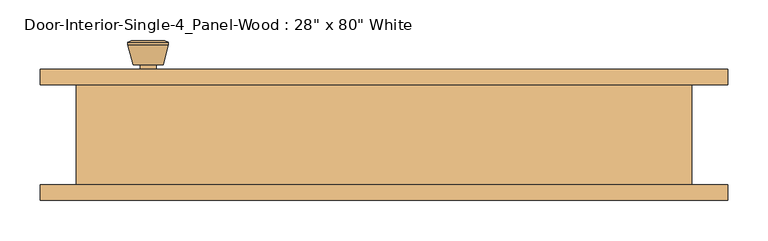
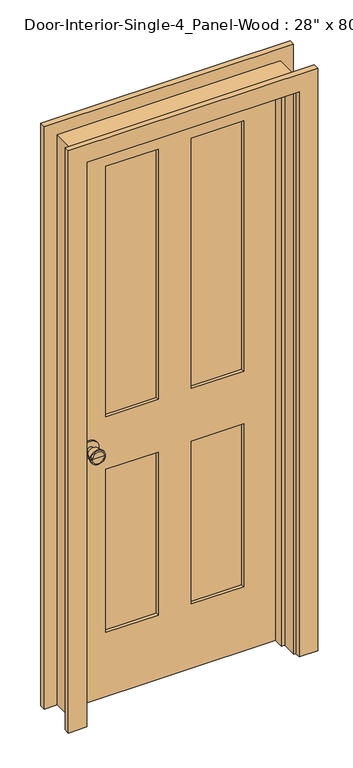
"""IFC4 building model written with IfcOpenShell, lengths in millimetres: door geometry."""

from ifc_helpers import new_model, si_unit, point, frame, frame_2d, origin, place, context, project, spatial, polyline, circle_curve, trimmed, segment, composite_curve, outline, extrude, faceted_brep, source, transform, mapped, element, save
from ifc_brep_helpers import plane_surface, cylinder_surface, revolved_surface, advanced_brep


def door_ede893c7(model_context):
    return source(origin(), model_context, "Body", "SolidModel", [
        advanced_brep(
        [(-292.1, 17.8125, 914.4), (-282.1, 17.8125, 914.4), (-302.1, 17.8125, 914.4), (-271.6241324, -31.1875, 914.4), (-292.1, -31.1875, 914.4), (-312.5758676, -31.1875, 914.4), (-267.1, -29.3596319, 914.4), (-317.1, -29.3596319, 914.4), (-267.1, -25.8959537, 914.4), (-317.1, -25.8959537, 914.4), (-273.463764, -1.1875, 914.4), (-310.736236, -1.1875, 914.4), (-282.1, -1.1875, 914.4), (-302.1, -1.1875, 914.4)],
        [
            (0, 1),
            (1, 2, circle_curve(frame((-292.1, 17.8125, 914.4), z_axis=(0.0, 1.0, 0.0), x_axis=(-1.0, 0.0, 0.0)), 10.0)),
            (2, 0),
            (2, 1, circle_curve(frame((-292.1, 17.8125, 914.4), z_axis=(0.0, 1.0, 0.0), x_axis=(-1.0, 0.0, 0.0)), 10.0)),
            (3, 4),
            (4, 5),
            (5, 3, circle_curve(frame((-292.1, -31.1875, 914.4), z_axis=(0.0, -1.0, 0.0), x_axis=(-1.0, 0.0, 0.0)), 20.4758676)),
            (3, 5, circle_curve(frame((-292.1, -31.1875, 914.4), z_axis=(0.0, -1.0, 0.0), x_axis=(-1.0, 0.0, 0.0)), 20.4758676)),
            (6, 3),
            (5, 7),
            (7, 6, circle_curve(frame((-292.1, -29.3596319, 914.4), z_axis=(0.0, -1.0, 0.0), x_axis=(-1.0, 0.0, 0.0)), 25.0)),
            (6, 7, circle_curve(frame((-292.1, -29.3596319, 914.4), z_axis=(0.0, -1.0, 0.0), x_axis=(-1.0, 0.0, 0.0)), 25.0)),
            (8, 6),
            (7, 9),
            (9, 8, circle_curve(frame((-292.1, -25.8959537, 914.4), z_axis=(0.0, -1.0, 0.0), x_axis=(-1.0, 0.0, 0.0)), 25.0)),
            (8, 9, circle_curve(frame((-292.1, -25.8959537, 914.4), z_axis=(0.0, -1.0, 0.0), x_axis=(-1.0, 0.0, 0.0)), 25.0)),
            (10, 8),
            (9, 11),
            (11, 10, circle_curve(frame((-292.1, -1.1875, 914.4), z_axis=(0.0, -1.0, 0.0), x_axis=(-1.0, 0.0, 0.0)), 18.636236)),
            (10, 11, circle_curve(frame((-292.1, -1.1875, 914.4), z_axis=(0.0, -1.0, 0.0), x_axis=(-1.0, 0.0, 0.0)), 18.636236)),
            (12, 10),
            (11, 13),
            (13, 12, circle_curve(frame((-292.1, -1.1875, 914.4), z_axis=(0.0, -1.0, 0.0), x_axis=(-1.0, 0.0, 0.0)), 10.0)),
            (12, 13, circle_curve(frame((-292.1, -1.1875, 914.4), z_axis=(0.0, -1.0, 0.0), x_axis=(-1.0, 0.0, 0.0)), 10.0)),
            (1, 12),
            (13, 2),
        ],
        [
            plane_surface(frame((-292.1, 17.8125, 914.4), z_axis=(0.0, 1.0, 0.0), x_axis=(-1.0, 0.0, 0.0))),
            plane_surface(frame((-292.1, -31.1875, 914.4), z_axis=(0.0, -1.0, 0.0), x_axis=(-1.0, 0.0, 0.0))),
            revolved_surface(polyline([(-312.5758676, -31.1875, 914.4), (-317.1, -29.3596319, 914.4)]), (-292.1, 17.8125, 914.4), (0.0, 1.0, 0.0)),
            cylinder_surface(frame((-292.1, 17.8125, 914.4), z_axis=(0.0, 1.0, 0.0), x_axis=(-1.0, 0.0, 0.0)), 25.0),
            revolved_surface(polyline([(-317.1, -25.8959537, 914.4), (-310.736236, -1.1875, 914.4)]), (-292.1, 17.8125, 914.4), (0.0, 1.0, 0.0)),
            plane_surface(frame((-292.1, -1.1875, 914.4), z_axis=(0.0, 1.0, 0.0), x_axis=(-1.0, 0.0, 0.0))),
            cylinder_surface(frame((-292.1, 17.8125, 914.4), z_axis=(0.0, 1.0, 0.0), x_axis=(-1.0, 0.0, 0.0)), 10.0),
        ],
        [
            (0, [[1, 2, 3]]),
            (0, [[-3, 4, -1]]),
            (1, [[5, 6, 7]]),
            (1, [[-6, -5, 8]]),
            (2, [[9, -7, 10, 11]]),
            (2, [[-10, -8, -9, 12]]),
            (3, [[13, -11, 14, 15]]),
            (3, [[-14, -12, -13, 16]]),
            (4, [[17, -15, 18, 19]]),
            (4, [[-18, -16, -17, 20]]),
            (5, [[21, -19, 22, 23]]),
            (5, [[-22, -20, -21, 24]]),
            (6, [[25, -23, 26, -2]]),
            (6, [[-26, -24, -25, -4]]),
        ],
    ),
        extrude(outline(composite_curve([segment(trimmed(circle_curve(frame_2d((914.4, -292.1)), 30.0), [point((914.4, -322.1))], [point((914.4, -262.1))], False, "CARTESIAN"), True, "CONTINUOUS"), segment(trimmed(circle_curve(frame_2d((914.4, -292.1)), 30.0), [point((914.4, -262.1))], [point((914.4, -322.1))], False, "CARTESIAN"), True, "CONTINUOUS")], self_intersect=False)), frame((0.0, 17.8125, 0.0), z_axis=(0.0, 1.0, 0.0), x_axis=(0.0, 0.0, 1.0)), (0.0, 0.0, 1.0), 6.0),
        advanced_brep(
        [(-292.1, 64.7375, 914.4), (-302.1, 64.7375, 914.4), (-282.1, 64.7375, 914.4), (-271.6241324, 113.7375, 914.4), (-312.5758676, 113.7375, 914.4), (-292.1, 113.7375, 914.4), (-267.1, 111.9096319, 914.4), (-317.1, 111.9096319, 914.4), (-267.1, 108.4459537, 914.4), (-317.1, 108.4459537, 914.4), (-273.463764, 83.7375, 914.4), (-310.736236, 83.7375, 914.4), (-282.1, 83.7375, 914.4), (-302.1, 83.7375, 914.4)],
        [
            (0, 1),
            (1, 2, circle_curve(frame((-292.1, 64.7375, 914.4), z_axis=(0.0, -1.0, 0.0), x_axis=(-1.0, 0.0, 0.0)), 10.0)),
            (2, 0),
            (2, 1, circle_curve(frame((-292.1, 64.7375, 914.4), z_axis=(0.0, -1.0, 0.0), x_axis=(-1.0, 0.0, 0.0)), 10.0)),
            (3, 4, circle_curve(frame((-292.1, 113.7375, 914.4), z_axis=(0.0, 1.0, 0.0), x_axis=(-1.0, 0.0, 0.0)), 20.4758676)),
            (4, 5),
            (5, 3),
            (4, 3, circle_curve(frame((-292.1, 113.7375, 914.4), z_axis=(0.0, 1.0, 0.0), x_axis=(-1.0, 0.0, 0.0)), 20.4758676)),
            (6, 7, circle_curve(frame((-292.1, 111.9096319, 914.4), z_axis=(0.0, 1.0, 0.0), x_axis=(-1.0, 0.0, 0.0)), 25.0)),
            (7, 4),
            (3, 6),
            (7, 6, circle_curve(frame((-292.1, 111.9096319, 914.4), z_axis=(0.0, 1.0, 0.0), x_axis=(-1.0, 0.0, 0.0)), 25.0)),
            (8, 9, circle_curve(frame((-292.1, 108.4459537, 914.4), z_axis=(0.0, 1.0, 0.0), x_axis=(-1.0, 0.0, 0.0)), 25.0)),
            (9, 7),
            (6, 8),
            (9, 8, circle_curve(frame((-292.1, 108.4459537, 914.4), z_axis=(0.0, 1.0, 0.0), x_axis=(-1.0, 0.0, 0.0)), 25.0)),
            (10, 11, circle_curve(frame((-292.1, 83.7375, 914.4), z_axis=(0.0, 1.0, 0.0), x_axis=(-1.0, 0.0, 0.0)), 18.636236)),
            (11, 9),
            (8, 10),
            (11, 10, circle_curve(frame((-292.1, 83.7375, 914.4), z_axis=(0.0, 1.0, 0.0), x_axis=(-1.0, 0.0, 0.0)), 18.636236)),
            (12, 13, circle_curve(frame((-292.1, 83.7375, 914.4), z_axis=(0.0, 1.0, 0.0), x_axis=(-1.0, 0.0, 0.0)), 10.0)),
            (13, 11),
            (10, 12),
            (13, 12, circle_curve(frame((-292.1, 83.7375, 914.4), z_axis=(0.0, 1.0, 0.0), x_axis=(-1.0, 0.0, 0.0)), 10.0)),
            (1, 13),
            (12, 2),
        ],
        [
            plane_surface(frame((-292.1, 64.7375, 914.4), z_axis=(0.0, -1.0, 0.0), x_axis=(-1.0, 0.0, 0.0))),
            plane_surface(frame((-292.1, 113.7375, 914.4), z_axis=(0.0, 1.0, 0.0), x_axis=(-1.0, 0.0, 0.0))),
            revolved_surface(polyline([(-312.5758676, 113.7375, 914.4), (-317.1, 111.9096319, 914.4)]), (-292.1, 64.7375, 914.4), (0.0, -1.0, 0.0)),
            cylinder_surface(frame((-292.1, 64.7375, 914.4), z_axis=(0.0, -1.0, 0.0), x_axis=(-1.0, 0.0, 0.0)), 25.0),
            revolved_surface(polyline([(-317.1, 108.4459537, 914.4), (-310.736236, 83.7375, 914.4)]), (-292.1, 64.7375, 914.4), (0.0, -1.0, 0.0)),
            plane_surface(frame((-292.1, 83.7375, 914.4), z_axis=(0.0, -1.0, 0.0), x_axis=(-1.0, 0.0, 0.0))),
            cylinder_surface(frame((-292.1, 64.7375, 914.4), z_axis=(0.0, -1.0, 0.0), x_axis=(-1.0, 0.0, 0.0)), 10.0),
        ],
        [
            (0, [[1, 2, 3]]),
            (0, [[-3, 4, -1]]),
            (1, [[5, 6, 7]]),
            (1, [[8, -7, -6]]),
            (2, [[9, 10, -5, 11]]),
            (2, [[12, -11, -8, -10]]),
            (3, [[13, 14, -9, 15]]),
            (3, [[16, -15, -12, -14]]),
            (4, [[17, 18, -13, 19]]),
            (4, [[20, -19, -16, -18]]),
            (5, [[21, 22, -17, 23]]),
            (5, [[24, -23, -20, -22]]),
            (6, [[-2, 25, -21, 26]]),
            (6, [[-4, -26, -24, -25]]),
        ],
    ),
        extrude(outline(composite_curve([segment(trimmed(circle_curve(frame_2d((914.4, -292.1)), 30.0), [point((914.4, -322.1))], [point((914.4, -262.1))], False, "CARTESIAN"), True, "CONTINUOUS"), segment(trimmed(circle_curve(frame_2d((914.4, -292.1)), 30.0), [point((914.4, -262.1))], [point((914.4, -322.1))], False, "CARTESIAN"), True, "CONTINUOUS")], self_intersect=False)), frame((0.0, 58.7375, 0.0), z_axis=(0.0, 1.0, 0.0), x_axis=(0.0, 0.0, 1.0)), (0.0, 0.0, 1.0), 6.0),
        extrude(outline(polyline([(234.95, 35.4541667), (57.15, 35.4541667), (57.15, 47.0958333), (234.95, 47.0958333), (234.95, 35.4541667)])), frame((0.0, 0.0, 1009.65), z_axis=(0.0, 0.0, 1.0), x_axis=(1.0, 0.0, 0.0)), (0.0, 0.0, 1.0), 903.2875),
        extrude(outline(polyline([(-57.15, 35.4541667), (-234.95, 35.4541667), (-234.95, 47.0958333), (-57.15, 47.0958333), (-57.15, 35.4541667)])), frame((0.0, 0.0, 1009.65), z_axis=(0.0, 0.0, 1.0), x_axis=(1.0, 0.0, 0.0)), (0.0, 0.0, 1.0), 903.2875),
        extrude(outline(polyline([(234.95, 35.4541667), (57.15, 35.4541667), (57.15, 47.0958333), (234.95, 47.0958333), (234.95, 35.4541667)])), frame((0.0, 0.0, 231.775), z_axis=(0.0, 0.0, 1.0), x_axis=(1.0, 0.0, 0.0)), (0.0, 0.0, 1.0), 587.375),
        extrude(outline(polyline([(-57.15, 35.4541667), (-234.95, 35.4541667), (-234.95, 47.0958333), (-57.15, 47.0958333), (-57.15, 35.4541667)])), frame((0.0, 0.0, 231.775), z_axis=(0.0, 0.0, 1.0), x_axis=(1.0, 0.0, 0.0)), (0.0, 0.0, 1.0), 587.375),
        extrude(outline(polyline([(2032.0, -355.6), (0.0, -355.6), (0.0, 355.6), (2032.0, 355.6), (2032.0, -355.6)]), holes=[polyline([(1912.9375, 57.15), (1912.9375, 234.95), (1009.65, 234.95), (1009.65, 57.15), (1912.9375, 57.15)]), polyline([(1009.65, -57.15), (1009.65, -234.95), (1912.9375, -234.95), (1912.9375, -57.15), (1009.65, -57.15)]), polyline([(819.15, 57.15), (819.15, 234.95), (231.775, 234.95), (231.775, 57.15), (819.15, 57.15)]), polyline([(231.775, -57.15), (231.775, -234.95), (819.15, -234.95), (819.15, -57.15), (231.775, -57.15)])]), frame((0.0, 23.8125, 0.0), z_axis=(0.0, 1.0, 0.0), x_axis=(0.0, 0.0, 1.0)), (0.0, 0.0, 1.0), 34.925),
        faceted_brep([(381.0, 58.7375, 0.0), (381.0, -65.0875, 0.0), (355.6, -65.0875, 0.0), (355.6, -11.1125, 0.0), (342.9, -11.1125, 0.0), (342.9, 23.8125, 0.0), (355.6, 23.8125, 0.0), (355.6, 58.7375, 0.0), (381.0, 58.7375, 2057.4), (381.0, -65.0875, 2057.4), (-381.0, -65.0875, 2057.4), (-381.0, -65.0875, 0.0), (-355.6, -65.0875, 0.0), (-355.6, -65.0875, 2032.0), (355.6, -65.0875, 2032.0), (355.6, -11.1125, 2032.0), (-355.6, -11.1125, 2032.0), (-355.6, -11.1125, 0.0), (-342.9, -11.1125, 0.0), (-342.9, -11.1125, 2019.3), (342.9, -11.1125, 2019.3), (342.9, 23.8125, 2019.3), (-342.9, 23.8125, 2019.3), (-342.9, 23.8125, 0.0), (-355.6, 23.8125, 0.0), (-355.6, 23.8125, 2032.0), (355.6, 23.8125, 2032.0), (355.6, 58.7375, 2032.0), (-355.6, 58.7375, 2032.0), (-355.6, 58.7375, 0.0), (-381.0, 58.7375, 0.0), (-381.0, 58.7375, 2057.4)], [[[0, 1, 2, 3, 4, 5, 6, 7]], [[1, 0, 8, 9]], [[2, 1, 9, 10, 11, 12, 13, 14]], [[3, 2, 14, 15]], [[4, 3, 15, 16, 17, 18, 19, 20]], [[5, 4, 20, 21]], [[6, 5, 21, 22, 23, 24, 25, 26]], [[7, 6, 26, 27]], [[0, 7, 27, 28, 29, 30, 31, 8]], [[9, 8, 31, 10]], [[15, 14, 13, 16]], [[21, 20, 19, 22]], [[27, 26, 25, 28]], [[30, 29, 24, 23, 18, 17, 12, 11]], [[10, 31, 30, 11]], [[16, 13, 12, 17]], [[22, 19, 18, 23]], [[28, 25, 24, 29]]]),
        extrude(outline(polyline([(0.0, 361.95), (0.0, 425.45), (2101.85, 425.45), (2101.85, -425.45), (0.0, -425.45), (0.0, -361.95), (2038.35, -361.95), (2038.35, 361.95), (0.0, 361.95)])), frame((0.0, -84.1375, 0.0), z_axis=(0.0, 1.0, 0.0), x_axis=(0.0, 0.0, 1.0)), (0.0, 0.0, 1.0), 19.05),
        extrude(outline(polyline([(0.0, 361.95), (0.0, 425.45), (2101.85, 425.45), (2101.85, -425.45), (0.0, -425.45), (0.0, -361.95), (2038.35, -361.95), (2038.35, 361.95), (0.0, 361.95)])), frame((0.0, 58.7375, 0.0), z_axis=(0.0, 1.0, 0.0), x_axis=(0.0, 0.0, 1.0)), (0.0, 0.0, 1.0), 19.05),
    ])


if __name__ == "__main__":
    model = new_model("IFC4")
    model_context = context("Model", 3, world=origin())
    ifc_project = project(units=[si_unit("LENGTHUNIT", "METRE", prefix="MILLI")], contexts=[model_context])
    site = spatial("IfcSite", under=ifc_project)
    building = spatial("IfcBuilding", under=site)
    placement = place(None, origin())
    door_shape = door_ede893c7(model_context)
    element("IfcDoor", 1, ObjectType="Door-Interior-Single-4_Panel-Wood : 28\" x 80\" White", at=placement, inside=building, context=model_context, shape_type="MappedRepresentation", body=[
        mapped(door_shape, transform((0.0, 0.0, 0.0), x_axis=(1.0, 0.0, 0.0), y_axis=(0.0, 1.0, 0.0), z_axis=(0.0, 0.0, 1.0))),
    ])
    save(model, "model.ifc")

# Revit data of these elements
# Type "Door-Interior-Single-4_Panel-Wood : 28\" x 80\" White"
#   Type Mark = "72"
#   COBie.Type.CreatedBy = "doug.wood@us.ibm.com"
#   COBie.Type.CreatedOn = "2016-04-14T02:07:24"
#   COBie.Type.Name = "Doors_Door-Interior-Single-4_Panel-Wood_28\" x 80\" White_72"
#   COBie.Type.Category = "23-30 10 00 : Doors"
#   COBie.Type.Description = "Door-Interior-Single-4_Panel-Wood_28\" x 80\" White"
#   COBie.Type.Manufacturer = ""
#   COBie.Type.ModelNumber = ""
#   Assembly Code = "C1020300"
#   Analytic Construction = "Wooden"
#   COBie.Type.ReplacementCost = 0
#   Top Rail = 0' - 4 11/16"
#   Thickness = 0' - 1 3/8"
#   Thermal Resistance (R) = 0.455703 (m²·K)/W
#   Swing Angle [instance default] = 90.00°
#   Stiles = 0' - 4 3/4"
#   Rough Width = 2' - 6"
#   Rough Height = 6' - 9"
#   Mullion = 0' - 4 1/2"
#   Lock Rail = 0' - 7 1/2"
#   Height = 6' - 8"
#   Width = 2' - 4"
#   Heat Transfer Coefficient (U) = 2.19465 W/(m²·K)
#   Bottom Rail = 0' - 9 1/8"
#   COBie.Type = no
#   Trim Material = Trim - White
#   Panel Material = Door - Panel - White
#   Frame Material = Door - Panel - White
#   Door Handle Material = ARCAT - Metal - Brass, Polished
#   Visual Light Transmittance = 0
#   Solar Heat Gain Coefficient = 0
#   Wall Closure = (empty or 0)
#   Function = (empty or 0)
# Element 1 (IfcDoor, "Door-Interior-Single-4_Panel-Wood : 28\" x 80\" White")
#   Materials on its faces: "Door - Panel - White", "ARCAT - Metal - Brass, Polished", "Trim - White"
# Materials
#   "Trim - White": class "Wood", colour RGB 255 255 255, transparency 0, Cost = 0
#   "Door - Panel - White": class "Wood", colour RGB 255 255 255, transparency 0, Cost = 0
#   "ARCAT - Metal - Brass, Polished": class "Unassigned", colour RGB 246 240 166, transparency 0, Keynote = "05050", Model = "Generic", Manufacturer = "Generic", Description = "Steel, Chrome Plated"
